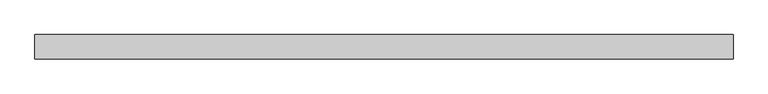
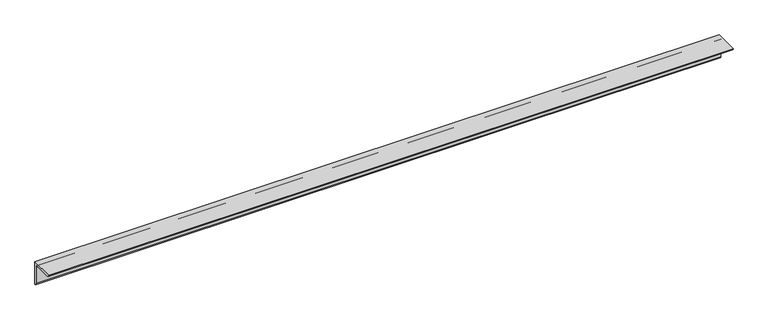
"""IFC4 building model written with IfcOpenShell, lengths in millimetres: member geometry, 0912_Steel Framing_L-KSD3502 : H_SB_AR_S03_L-130x130x12_HBR3."""

from ifc_helpers import new_model, si_unit, point, frame, frame_2d, origin, place, context, project, spatial, polyline, circle_curve, trimmed, segment, composite_curve, outline, extrude, source, transform, mapped, element, save


def member_277812e4(model_context):
    return source(origin(), model_context, "Body", "SweptSolid", [
        extrude(outline(composite_curve([segment(polyline([(36.4, 36.4), (36.4, -93.6)]), True, "CONTINUOUS"), segment(trimmed(circle_curve(frame_2d((36.4, -81.6)), 12.0), [point((36.4, -93.6))], [point((24.4, -81.6))], False, "CARTESIAN"), True, "CONTINUOUS"), segment(polyline([(24.4, -81.6), (24.4, 12.4)]), True, "CONTINUOUS"), segment(trimmed(circle_curve(frame_2d((12.4, 12.4)), 12.0), [point((24.4, 12.4))], [point((12.4, 24.4))], True, "CARTESIAN"), True, "CONTINUOUS"), segment(polyline([(12.4, 24.4), (-81.6, 24.4)]), True, "CONTINUOUS"), segment(trimmed(circle_curve(frame_2d((-81.6, 36.4)), 12.0), [point((-81.6, 24.4))], [point((-93.6, 36.4))], False, "CARTESIAN"), True, "CONTINUOUS"), segment(polyline([(-93.6, 36.4), (36.4, 36.4)]), True, "CONTINUOUS")], self_intersect=False)), frame((-1852.8554237, 0.0, 0.0), z_axis=(1.0, 0.0, 0.0), x_axis=(0.0, 1.0, 0.0)), (0.0, 0.0, 1.0), 3720.541926),
    ])


if __name__ == "__main__":
    model = new_model("IFC4")
    model_context = context("Model", 3, world=origin())
    ifc_project = project(units=[si_unit("LENGTHUNIT", "METRE", prefix="MILLI")], contexts=[model_context])
    site = spatial("IfcSite", under=ifc_project)
    building = spatial("IfcBuilding", under=site)
    placement = place(None, origin())
    member_shape = member_277812e4(model_context)
    element("IfcMember", 1, ObjectType="0912_Steel Framing_L-KSD3502 : H_SB_AR_S03_L-130x130x12_HBR3", at=placement, inside=building, context=model_context, shape_type="MappedRepresentation", body=[
        mapped(member_shape, transform((0.0, 0.0, 0.0), x_axis=(1.0, 0.0, 0.0), y_axis=(0.0, 1.0, 0.0), z_axis=(0.0, 0.0, 1.0))),
    ])
    save(model, "model.ifc")

# Revit data of these elements
# Type "0912_Steel Framing_L-KSD3502 : H_SB_AR_S03_L-130x130x12_HBR3"
#   k = 25 mm
#   Perimeter = 0.52 m²/m
#   Nominal Weight = 23.40 kgf/m
#   Length [instance default] = 1000 mm
#   b = 130 mm
#   d = 130 mm
#   t = 12 mm
#   x = 36.4 mm
#   y = 36.4 mm
#   A = 2976.00 m²
#   Structural Material [instance default] = Steel, 45-345
# Element 1 (IfcMember, "0912_Steel Framing_L-KSD3502 : H_SB_AR_S03_L-130x130x12_HBR3")
#   Structural Material = Steel ASTM A36
#   Materials on its faces: "Steel ASTM A36"
# Materials
#   "Steel, 45-345": class "Metal", colour RGB 189 187 185, transparency 0, Description = "Steel 345 MPa", Cost = 0
#   "Steel ASTM A36": class "Metal", colour RGB 199 199 199, transparency 0, Description = "Structural steel, ASTM A36 Grade B, mill finish", Cost = 0
